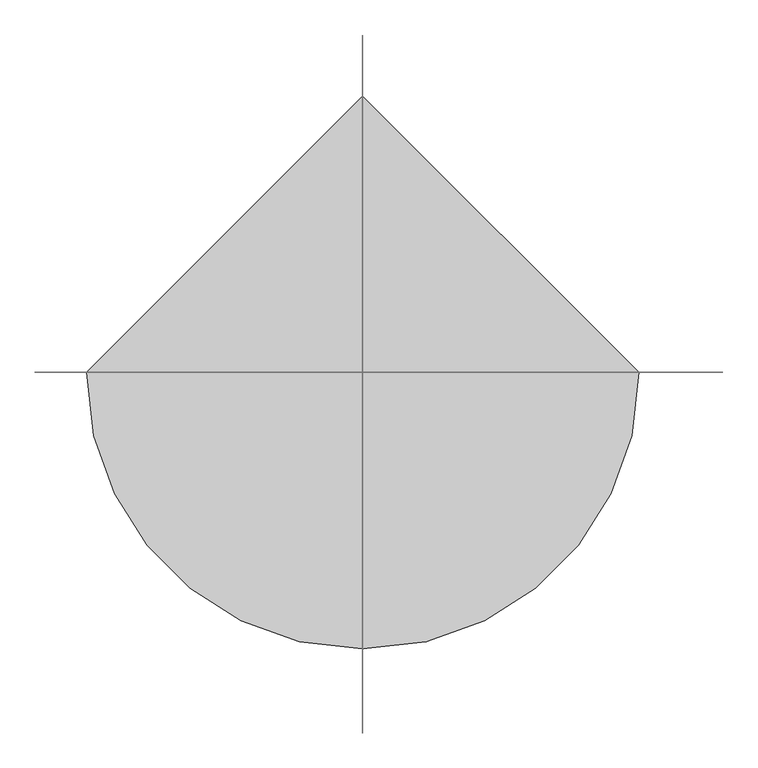
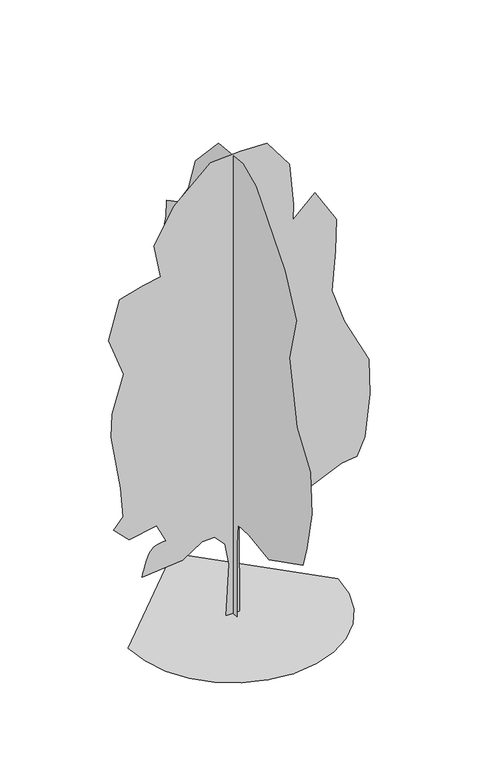
"""IFC4 building model written with IfcOpenShell, lengths in millimetres: geographic element geometry, RPC 木 - 落葉樹 : レッド アッシュ - 7.6 メートル."""

from ifc_helpers import new_model, si_unit, origin, place, context, project, spatial, triangles, source, transform, mapped, element, save


def geographic_element_16c8020d(model_context):
    return source(origin(), model_context, "Body", "Tessellation", [
        triangles([(-1640.6350319, 0.0, 6.17e-05), (-1597.2618073, -375.9250554, 6.17e-05), (-1473.7362076, -721.1521299, 6.17e-05), (-1279.9481815, -1025.7899305, 6.17e-05), (-1025.7900759, -1279.9483269, 6.17e-05), (-721.1519119, -1473.7357716, 6.17e-05), (-375.9249101, -1597.2618073, 6.17e-05), (7.17e-05, -1640.6350319, 6.17e-05), (375.9250917, -1597.2619526, 6.17e-05), (721.1521299, -1473.7360622, 6.17e-05), (1025.7900759, -1279.9481815, 6.17e-05), (1279.9486176, -1025.7900759, 6.17e-05), (1473.7359169, -721.1518393, 6.17e-05), (1597.2618073, -375.9248011, 6.17e-05), (1640.6350319, 0.0001434, 6.17e-05), (-0.0002151, 1640.6350319, 6.17e-05), (-1.07e-05, -102.5763152, 0.0), (2.5e-05, -100.9809819, 1191.4187742), (3.22e-05, -129.5410573, 1533.7667004), (7e-07, -437.6736119, 1554.0757805), (-5.76e-05, -973.8285673, 1474.4268631), (-0.0001401, -1898.6961697, 1943.5624718), (-0.0001409, -2005.9272697, 2292.063438), (-0.0001357, -2139.9660358, 2935.4493118), (-0.0001116, -2099.7546822, 3605.6435783), (-5.8e-05, -1735.814106, 4130.1484818), (-5.5e-06, -1523.3897175, 5147.0898972), (-3.5e-06, -1711.0423622, 5870.899205), (4.78e-05, -1402.7536217, 6514.2855148), (0.0001565, -625.3287638, 7439.1534805), (0.000198, -272.4836404, 7598.1990051), (0.0002655, 393.3664327, 7532.9808929), (0.0003113, 1023.3488731, 6862.7869171), (0.0003141, 1211.0034073, 6299.8236053), (0.0003314, 1492.4837551, 5897.706871), (0.0003588, 1800.7742397, 5736.8608749), (0.0003522, 1814.1780727, 5468.7830521), (0.0003514, 1894.6015068, 5160.4937302), (0.0003267, 1760.5627407, 4798.5890762), (0.0003288, 1881.1975285, 4450.088546), (0.000327, 2001.8324615, 3967.5488136), (0.0003203, 1975.0247955, 3833.5096115), (0.0002869, 1747.159053, 3511.8164566), (0.0002722, 1732.7516476, 3069.4885139), (0.0002625, 1720.3510963, 2788.0068581), (0.0002535, 1733.7549294, 2439.5063278), (0.0002406, 1747.159053, 1956.9668861), (0.0002166, 1559.5045189, 1809.523851), (0.0001802, 1211.0038433, 1809.523851), (0.0001822, 1371.8504208, 1313.580431), (0.0001711, 1344.9556961, 1032.1683203), (0.0001512, 1100.1359739, 1224.6137684), (9.84e-05, 627.810589, 1103.8028286), (9.77e-05, 550.2637599, 1353.49907), (6.27e-05, 215.346067, 1350.4488201), (5.01e-05, 130.4579254, 1225.1105404), (3.26e-05, 79.3405423, 816.1354311), (1.17e-05, 111.8716144, 1.28e-05), (-110.5798692, 4.8e-06, 4.45e-05), (-66.5363775, -9.62e-05, 831.3140104), (-128.9679092, -0.0001356, 1184.825572), (-290.0246482, -0.0001497, 1361.7341778), (-482.3670685, -0.0001405, 1355.1302204), (-794.1778324, -0.0001027, 1152.7338535), (-1424.1601639, -6.88e-05, 1099.1184488), (-1415.4458702, -7.33e-05, 1133.7810133), (-1406.1451298, -7.8e-05, 1169.6158899), (-1395.6722225, -8.3e-05, 1207.7952456), (-1383.4407017, -8.85e-05, 1249.4921917), (-1368.8645565, -9.46e-05, 1295.8774418), (-1351.3574856, -0.0001016, 1348.1257061), (-1330.3333328, -0.0001096, 1407.4074074), (-1303.8382931, -0.0001173, 1462.3908245), (-1271.0123898, -0.0001236, 1502.6024689), (-1232.9109364, -0.0001286, 1530.5039635), (-1190.588883, -0.0001326, 1548.5586754), (-1145.1018339, -0.0001358, 1559.2267742), (-1097.5041578, -0.0001386, 1564.971191), (-1048.8515316, -0.0001411, 1568.2539848), (-1196.294058, -0.0001698, 1863.1393284), (-1625.218531, -0.0001415, 1782.7160397), (-1866.4879612, -0.0001597, 2023.9861965), (-1719.0452168, -0.0001869, 2198.236607), (-1759.2568611, -0.0002427, 2680.7764847), (-1906.6994602, -0.0003433, 3578.8359123), (-1893.4979404, -0.0003882, 3950.7687332), (-1715.4032879, -0.0004676, 4551.3483536), (-1946.9112499, -0.0005333, 5187.3013962), (-1772.6605488, -0.0006144, 5803.88004), (-1410.7561855, -0.000643, 5911.1112854), (-1135.4252443, -0.0006608, 5959.6792511), (-1236.5059204, -0.0007209, 6500.8816818), (-928.2163805, -0.0007999, 7050.4411606), (-351.8493811, -0.0008874, 7573.192392), (117.2860368, -0.0009111, 7600.000058), (532.8066133, -0.0009277, 7586.5956436), (881.3074705, -0.000887, 7117.4603256), (945.3842279, -0.0008079, 6430.5952744), (936.1832634, -0.0007775, 6178.7100677), (1283.4236961, -0.0008311, 6500.8816818), (1618.5208294, -0.0007802, 5951.3222031), (1605.1169964, -0.0007177, 5432.2143539), (1545.3907001, -0.0006383, 4788.0519287), (1739.1557625, -0.0005793, 4222.2222221), (2126.1689129, -0.0005054, 3460.0925789), (2138.5076946, -0.0004374, 2885.2169128), (2060.8486267, -0.0003521, 2198.2364616), (1940.213839, -0.0003133, 1916.7548058), (1698.9439728, -0.0002996, 1889.9471397), (1229.8082188, -0.0002535, 1675.4849396), (814.2876514, -0.0002002, 1380.5997414), (256.8007496, -0.0002044, 1620.3048775), (92.8066444, -0.0001762, 1443.8352711), (103.8818677, -4.5e-06, 3.51e-05)], [[15, 16, 1], [14, 15, 1], [14, 1, 2], [13, 14, 2], [13, 2, 3], [13, 3, 4], [12, 13, 4], [11, 12, 4], [11, 4, 5], [11, 5, 6], [11, 6, 7], [11, 7, 8], [11, 8, 9], [11, 9, 10], [50, 51, 52], [57, 58, 17], [57, 17, 18], [56, 57, 18], [56, 18, 19], [55, 56, 19], [49, 50, 52], [52, 53, 54], [49, 52, 54], [35, 36, 37], [46, 47, 48], [46, 48, 49], [21, 22, 23], [20, 21, 23], [20, 23, 24], [20, 24, 25], [20, 25, 26], [19, 20, 26], [19, 26, 27], [45, 46, 49], [31, 32, 33], [30, 31, 33], [29, 30, 33], [29, 33, 34], [28, 29, 34], [27, 28, 34], [19, 27, 34], [19, 34, 35], [19, 35, 37], [19, 37, 38], [19, 38, 39], [19, 39, 40], [19, 40, 41], [19, 41, 42], [19, 42, 43], [19, 43, 44], [19, 44, 45], [19, 45, 49], [19, 49, 54], [55, 19, 54], [64, 65, 66], [64, 66, 67], [64, 67, 68], [99, 100, 101], [64, 68, 69], [64, 69, 70], [64, 70, 71], [114, 59, 60], [113, 114, 60], [113, 60, 61], [113, 61, 62], [64, 71, 72], [64, 72, 73], [64, 73, 74], [64, 74, 75], [64, 75, 76], [64, 76, 77], [64, 77, 78], [64, 78, 79], [63, 64, 79], [81, 82, 83], [80, 81, 83], [99, 101, 102], [107, 108, 109], [110, 111, 112], [88, 89, 90], [87, 88, 90], [87, 90, 91], [80, 83, 84], [95, 96, 97], [95, 97, 98], [94, 95, 98], [93, 94, 98], [92, 93, 98], [91, 92, 98], [91, 98, 99], [87, 91, 99], [87, 99, 102], [87, 102, 103], [87, 103, 104], [86, 87, 104], [85, 86, 104], [84, 85, 104], [80, 84, 104], [80, 104, 105], [80, 105, 106], [80, 106, 107], [80, 107, 109], [80, 109, 110], [80, 110, 112], [79, 80, 112], [63, 79, 112], [62, 63, 112], [113, 62, 112]], closed=False),
    ])


if __name__ == "__main__":
    model = new_model("IFC4")
    model_context = context("Model", 3, world=origin())
    ifc_project = project(units=[si_unit("LENGTHUNIT", "METRE", prefix="MILLI")], contexts=[model_context])
    site = spatial("IfcSite", under=ifc_project)
    building = spatial("IfcBuilding", under=site)
    placement = place(None, origin())
    geographic_element_shape = geographic_element_16c8020d(model_context)
    element("IfcGeographicElement", 1, ObjectType="RPC 木 - 落葉樹 : レッド アッシュ - 7.6 メートル", at=placement, inside=building, context=model_context, shape_type="MappedRepresentation", body=[
        mapped(geographic_element_shape, transform((0.0, 0.0, 0.0), x_axis=(1.0, 0.0, 0.0), y_axis=(0.0, 1.0, 0.0), z_axis=(0.0, 0.0, 1.0))),
    ])
    save(model, "model.ifc")

# Revit data of these elements
# Type "RPC 木 - 落葉樹 : レッド アッシュ - 7.6 メートル"
#   built-in parameter 1005198 = "{2, 15},{22, RPC-8-G3GR-497X-PHW5-6},{1, 0},{1, 0},{2, 37},{1, 8},{5, Color},{1, 0},{1, 0},{3, 0.8},{3, 0.8},{3, 0.8},{1, 8},{7, BBoxMin},{1, 0},{1, 0},{1, 0},{1, 0},{1, 0},{1, 8},{7, BBoxMax},{1, 0},{1, 0},{1, 0},{1, 0},{1, 0},{2, 11},{9, RPCTypeId},{1, 0},{1, 0},{22, RPC-8-G3GR-497X-PHW5-6},{1, 6},{14, RPCPlantHeight},{1, 0},{1, 0},{7, 24.9344},{2, 11},{7, keyword},{1, 0},{1, 0},{78, :Geometry:RPC:Red Ash:red ash:frainus pennsylvanica:frene rouge:deciduous:tree},{2, 11},{8, category},{1, 0},{1, 0},{16, :Trees [General]},{2, 11},{12, LocalizedUID},{1, 0},{1, 0},{7, Red Ash},{2, 14},{6, Height},{1, 0},{1, 0},{7, 24.9344},{1, 2},{16, Cast Reflections},{1, 0},{1, 0},{1, 0},{1, 2},{6, Jitter},{1, 0},{1, 0},{1, 1},{1, 2},{9, Billboard},{1, 0},{1, 0},{1, 0},{1, 2},{12, Cast Shadows},{1, 0},{1, 0},{1, 1},{1, 2},{20, Apply Filter Effects},{1, 0},{1, 0},{1, 0},{2, 11},{28, Apply Filter Effects-Text-FC},{1, 0},{1, 0},{4, None},{2, 11},{20, AdvancedUIDefinition},{1, 0},{1, 0},{0, },{2, 11},{10, AssetLibID},{1, 0},{1, 0},{36, 4D3F6E72-3F99-4203-98E9-AF80B3C7A7A4},{2, 11},{10, BaseSchema},{1, 0},{1, 0},{9, RPCSchema},{2, 11},{12, ExchangeGUID},{1, 0},{1, 0},{0, },{1, 2},{6, Hidden},{1, 0},{1, 0},{1, 0},{1, 4},{11, RPCCategory},{1, 0},{1, 0},{1, 0},{2, 11},{8, RPCImage},{1, 0},{1, 0},{0, },{1, 4},{13, SchemaVersion},{1, 0},{1, 0},{1, 4},{2, 11},{12, UIDefinition},{1, 0},{1, 0},{0, },{2, 11},{6, UIName},{1, 0},{1, 0},{22, RPC-8-G3GR-497X-PHW5-6},{2, 11},{11, VersionGUID},{1, 0},{1, 0},{9, RPCSchema},{2, 11},{9, assettype},{1, 0},{1, 0},{11, RPCGeometry},{2, 11},{11, description},{1, 0},{1, 0},{0, },{2, 11},{9, localname},{1, 0},{1, 0},{3, RPC},{2, 11},{9, localtype},{1, 0},{1, 0},{3, RPC},{1, 4},{8, revision},{1, 0},{1, 0},{1, 1},{2, 11},{9, thumbnail},{1, 0},{1, 0},{0, },{1, 4},{7, version},{1, 0},{1, 0},{1, 1},{1, 2},{20, RPC_Cast Reflections},{1, 0},{1, 0},{1, 1},{1, 2},{10, RPC_Jitter},{1, 0},{1, 0},{1, 1},{1, 2},{13, RPC_Billboard},{1, 0},{1, 0},{1, 0},{1, 2},{16, RPC_Cast Shadows},{1, 0},{1, 0},{1, 1},{21, assetlibrary_base.fbx},{1, 5},"
#   built-in parameter 1005195 = "RPC-8-G3GR-497X-PHW5-6"
#   Type Comments = "レッド アッシュ"
#   Height = 7600 mm
#   Default Elevation = 0
